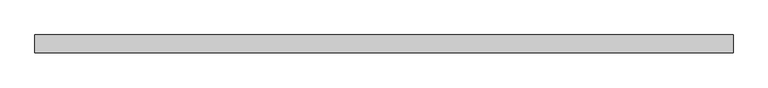
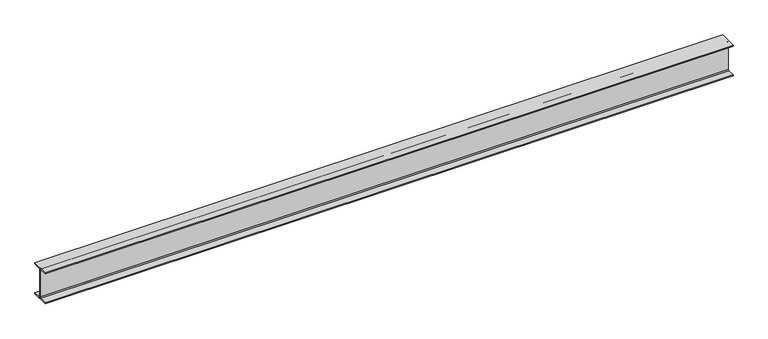
"""IFC4 building model written with IfcOpenShell, lengths in millimetres: beam geometry, Old_Steel Beam_H-KSD3502 : H_SB_ASB_H-390×300x10x16."""

from ifc_helpers import new_model, si_unit, point, frame, frame_2d, origin, place, context, project, spatial, polyline, circle_curve, trimmed, segment, composite_curve, outline, extrude, source, transform, mapped, element, save


def beam_21e8d8f4(model_context):
    return source(origin(), model_context, "Body", "SweptSolid", [
        extrude(outline(composite_curve([segment(polyline([(82.5, -141.5), (82.5, -151.7), (-82.5, -151.7), (-82.5, -141.5), (-11.9, -141.5)]), True, "CONTINUOUS"), segment(trimmed(circle_curve(frame_2d((-11.9, -132.6)), 8.9), [point((-11.9, -141.5))], [point((-3.0, -132.6))], True, "CARTESIAN"), True, "CONTINUOUS"), segment(polyline([(-3.0, -132.6), (-3.0, 132.6)]), True, "CONTINUOUS"), segment(trimmed(circle_curve(frame_2d((-11.9, 132.6)), 8.9), [point((-3.0, 132.6))], [point((-11.9, 141.5))], True, "CARTESIAN"), True, "CONTINUOUS"), segment(polyline([(-11.9, 141.5), (-82.5, 141.5), (-82.5, 151.7), (82.5, 151.7), (82.5, 141.5), (11.9, 141.5)]), True, "CONTINUOUS"), segment(trimmed(circle_curve(frame_2d((11.9, 132.6)), 8.9), [point((11.9, 141.5))], [point((3.0, 132.6))], True, "CARTESIAN"), True, "CONTINUOUS"), segment(polyline([(3.0, 132.6), (3.0, -132.6)]), True, "CONTINUOUS"), segment(trimmed(circle_curve(frame_2d((11.9, -132.6)), 8.9), [point((3.0, -132.6))], [point((11.9, -141.5))], True, "CARTESIAN"), True, "CONTINUOUS"), segment(polyline([(11.9, -141.5), (82.5, -141.5)]), True, "CONTINUOUS")], self_intersect=False)), frame((-3237.2999994, 0.0, 0.0), z_axis=(1.0, 0.0, 0.0), x_axis=(0.0, 1.0, 0.0)), (0.0, 0.0, 1.0), 6392.0999994),
    ])


if __name__ == "__main__":
    model = new_model("IFC4")
    model_context = context("Model", 3, world=origin())
    ifc_project = project(units=[si_unit("LENGTHUNIT", "METRE", prefix="MILLI")], contexts=[model_context])
    site = spatial("IfcSite", under=ifc_project)
    building = spatial("IfcBuilding", under=site)
    placement = place(None, origin())
    beam_shape = beam_21e8d8f4(model_context)
    element("IfcBeam", 1, ObjectType="Old_Steel Beam_H-KSD3502 : H_SB_ASB_H-390×300x10x16", at=placement, inside=building, context=model_context, shape_type="MappedRepresentation", body=[
        mapped(beam_shape, transform((0.0, 0.0, 0.0), x_axis=(1.0, 0.0, 0.0), y_axis=(0.0, 1.0, 0.0), z_axis=(0.0, 0.0, 1.0))),
    ])
    save(model, "model.ifc")

# Revit data of these elements
# Type "Old_Steel Beam_H-KSD3502 : H_SB_ASB_H-390×300x10x16"
#   Width = 30.0 cm
#   Web Thickness = 1.0 cm
#   Web Fillet = 2.2 cm
#   Warping Constant = 2517770.0 cm⁶
#   Torsional Moment of Inertia = 94.3867 cm⁴
#   Torsional Modulus = 1.0 cm³
#   Section Area = 136.0 cm²
#   Plastic Modulus weak axis = 733.0 cm³
#   Plastic Modulus strong axis = 2190.0 cm³
#   Perimeter = 1.92 m²/m
#   Nominal Weight = 107.00 kgf/m
#   Moment of Inertia weak axis = 7210.00 cm⁴
#   Moment of Inertia strong axis = 38700.00 cm⁴
#   Height = 39.0 cm
#   Flange Thickness = 1.6 cm
#   Elastic Modulus weak axis = 481.0 cm³
#   Elastic Modulus strong axis = 1980.0 cm³
#   Centroid Vertical = 19.5 cm
#   Centroid Horizontal = 15.0 cm
#   Length [instance default] = 1.5240 m
#   Structural Material [instance default] = Steel, 45-345
#   Assembly Code = ""
# Element 1 (IfcBeam, "Old_Steel Beam_H-KSD3502 : H_SB_ASB_H-390×300x10x16")
#   Structural Material = none
# Materials
#   "Steel, 45-345": class "Metal", colour RGB 189 187 185, transparency 0, Description = "Steel 345 MPa", Cost = 0
